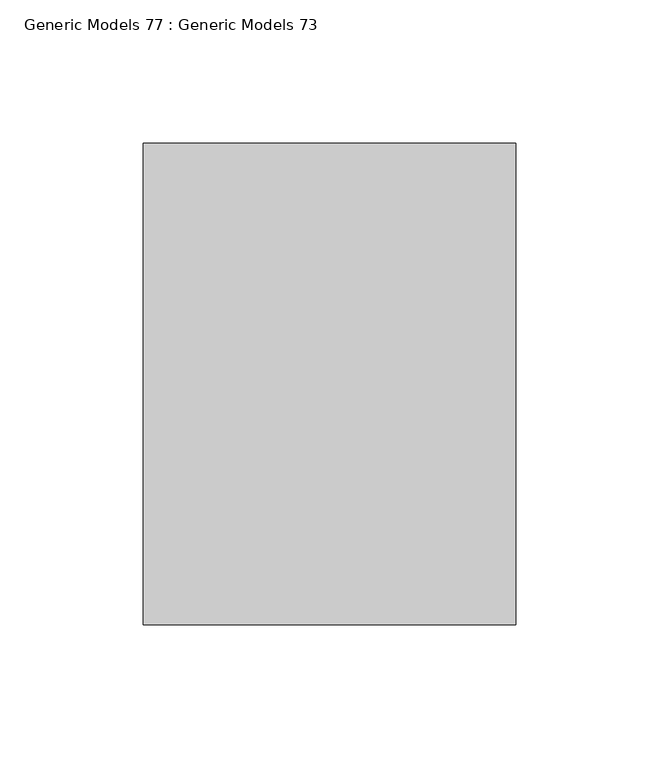
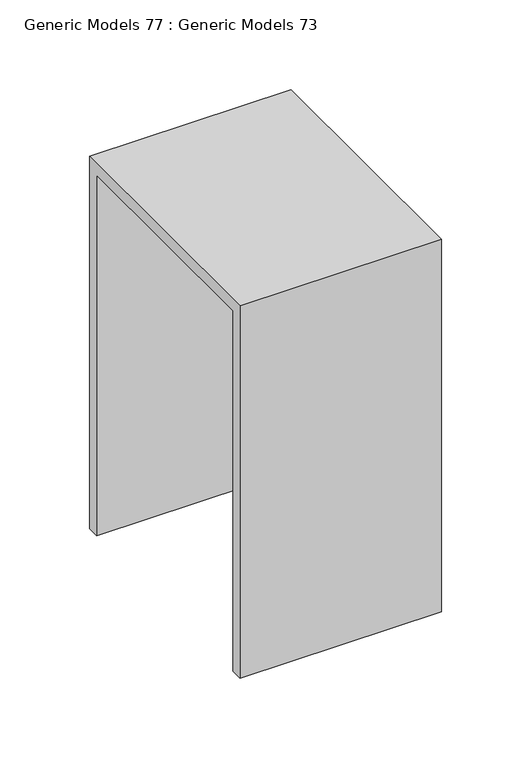
"""IFC4 building model written with IfcOpenShell, lengths in millimetres: proxy geometry, Generic Models 77 : Generic Models 73."""

import ifcopenshell
import ifcopenshell.guid

model = None  # the IFC model being written
_history = None  # IfcOwnerHistory: only IFC2X3 demands one
_inside = {}  # id of a spatial element -> (the spatial element, [elements in it])
_under = {}  # id of a project, library or spatial element -> (it, [spatial elements below it])
_declared = {}  # id of a project -> (the project, [libraries it declares])
_typed = {}  # id of a type object -> (the type object, [elements of that type])
_made_of = {}  # id of a material, layer set ... -> (it, [elements and type objects made of it])


def new_model(schema):
    """Start an empty IFC model of exactly this schema.

    Asked for "IFC4X3", IfcOpenShell would pick the latest addendum, in which some entities
    have other attributes; the version numbers below select the first issue.
    IFC2X3 requires an IfcOwnerHistory on every rooted entity: one is made here for all.
    """
    global model, _history
    if schema == "IFC4X3":
        model = ifcopenshell.file(schema_version=(4, 3, 0, 0))
    else:
        model = ifcopenshell.file(schema=schema)
    _inside.clear()
    _under.clear()
    _declared.clear()
    _typed.clear()
    _made_of.clear()
    _history = None
    if model.schema == "IFC2X3":
        org = make("IfcOrganization", Name="unknown")
        user = make(
            "IfcPersonAndOrganization",
            ThePerson=make("IfcPerson", FamilyName="unknown"),
            TheOrganization=org,
        )
        app = make(
            "IfcApplication",
            ApplicationDeveloper=org,
            Version="unknown",
            ApplicationFullName="unknown",
            ApplicationIdentifier="unknown",
        )
        _history = make(
            "IfcOwnerHistory",
            OwningUser=user,
            OwningApplication=app,
            ChangeAction="ADDED",
            CreationDate=0,
        )
    return model


def make(cls, **values):
    """One entity of the class cls with the attributes given. An attribute that is None is left unset."""
    return model.create_entity(
        cls, **{name: value for name, value in values.items() if value is not None}
    )


def rooted(cls, **values):
    """An entity with a GlobalId (a new one), such as an element, a storey or a relation."""
    return make(cls, GlobalId=ifcopenshell.guid.new(), OwnerHistory=_history, **values)


def si_unit(unit_type, name, prefix=None):
    """IfcSIUnit, for example si_unit("LENGTHUNIT", "METRE", prefix="MILLI")."""
    return make("IfcSIUnit", UnitType=unit_type, Prefix=prefix, Name=name)


def assignment(units):
    """IfcUnitAssignment: the units of a project."""
    return None if units is None else make("IfcUnitAssignment", Units=units)


def point(xyz):
    """IfcCartesianPoint."""
    return None if xyz is None else make("IfcCartesianPoint", Coordinates=xyz)


def direction(xyz):
    """IfcDirection."""
    return None if xyz is None else make("IfcDirection", DirectionRatios=xyz)


def frame(location, z_axis=None, x_axis=None):
    """IfcAxis2Placement3D, a coordinate frame: its origin and axes. An axis left out is left unset."""
    return make(
        "IfcAxis2Placement3D",
        Location=point(location),
        Axis=direction(z_axis),
        RefDirection=direction(x_axis),
    )


def origin():
    """The frame at (0, 0, 0) with its axes left unset."""
    return frame((0.0, 0.0, 0.0))


def place(relative_to, where):
    """IfcLocalPlacement: puts the frame where relative to a parent placement (None: the world)."""
    return make(
        "IfcLocalPlacement", PlacementRelTo=relative_to, RelativePlacement=where
    )


def context(
    kind, dimensions, precision=None, world=None, true_north=None, identifier=None
):
    """IfcGeometricRepresentationContext, for example the 3D "Model" context."""
    return make(
        "IfcGeometricRepresentationContext",
        ContextIdentifier=identifier,
        ContextType=kind,
        CoordinateSpaceDimension=dimensions,
        Precision=precision,
        WorldCoordinateSystem=world,
        TrueNorth=true_north,
    )


def project(units=None, contexts=None):
    """IfcProject with its units and contexts."""
    return rooted(
        "IfcProject",
        Name="project",
        RepresentationContexts=contexts,
        UnitsInContext=assignment(units),
    )


def spatial(cls, under=None, at=None, **own):
    """A site, building, storey or space (cls), placed at a placement, below another one or the project."""
    s = rooted(cls, ObjectPlacement=at, **own)
    if under is not None:
        _under.setdefault(under.id(), (under, []))[1].append(s)
    return s


def polyline(points):
    """IfcPolyline through the points."""
    return make("IfcPolyline", Points=[point(p) for p in points])


def outline(outer, holes=None, kind="AREA"):
    """IfcArbitraryClosedProfileDef: a profile drawn as a closed curve; with holes, ...WithVoids."""
    if holes is None:
        return make("IfcArbitraryClosedProfileDef", ProfileType=kind, OuterCurve=outer)
    return make(
        "IfcArbitraryProfileDefWithVoids",
        ProfileType=kind,
        OuterCurve=outer,
        InnerCurves=holes,
    )


def extrude(swept, where, along, depth):
    """IfcExtrudedAreaSolid: the profile swept, set in the frame where, extruded along a direction by depth."""
    return make(
        "IfcExtrudedAreaSolid",
        SweptArea=swept,
        Position=where,
        ExtrudedDirection=direction(along),
        Depth=depth,
    )


def shape(context_of_items, identifier, shape_type, items):
    """IfcShapeRepresentation: the items that make up one representation, for example the "Body"."""
    return make(
        "IfcShapeRepresentation",
        ContextOfItems=context_of_items,
        RepresentationIdentifier=identifier,
        RepresentationType=shape_type,
        Items=items,
    )


def source(mapping_origin, context_of_items, identifier, shape_type, items):
    """IfcRepresentationMap: a shape defined once, which mapped items show again and again."""
    return make(
        "IfcRepresentationMap",
        MappingOrigin=mapping_origin,
        MappedRepresentation=shape(context_of_items, identifier, shape_type, items),
    )


def transform(
    local_origin,
    x_axis=None,
    y_axis=None,
    z_axis=None,
    scale=None,
    scale2=None,
    scale3=None,
    uniform=True,
):
    """IfcCartesianTransformationOperator3D, or its non-uniform kind. x_axis, y_axis, z_axis: its Axis1, 2, 3."""
    if uniform:
        return make(
            "IfcCartesianTransformationOperator3D",
            Axis1=direction(x_axis),
            Axis2=direction(y_axis),
            LocalOrigin=point(local_origin),
            Scale=scale,
            Axis3=direction(z_axis),
        )
    return make(
        "IfcCartesianTransformationOperator3DnonUniform",
        Axis1=direction(x_axis),
        Axis2=direction(y_axis),
        LocalOrigin=point(local_origin),
        Scale=scale,
        Axis3=direction(z_axis),
        Scale2=scale2,
        Scale3=scale3,
    )


def mapped(mapping_source, mapping_target):
    """IfcMappedItem: shows the shape of a source again, moved by a transform."""
    return make(
        "IfcMappedItem", MappingSource=mapping_source, MappingTarget=mapping_target
    )


def made_of(thing, what):
    """Note that an element or type object is made of a material, layer set ...; save() writes the relation."""
    if what is not None:
        _made_of.setdefault(what.id(), (what, []))[1].append(thing)
    return thing


def element(
    cls,
    number,
    at=None,
    inside=None,
    cuts=None,
    type_object=None,
    material=None,
    context=None,
    identifier="Body",
    shape_type=None,
    held_by="IfcProductDefinitionShape",
    body=None,
    shapes=None,
    **own,
):
    """One element of the class cls, such as IfcWall. Its Tag is "e" and its number.

    at: its placement. inside: the storey or other place that contains it. cuts: it is an
    opening in that element (IfcRelVoidsElement). A single representation is given by context,
    identifier, shape_type and body (its items); several are given by shapes. held_by: the class
    of the entity that holds the representations. save() writes the other relations.
    """
    e = rooted(cls, Tag="e%d" % number, ObjectPlacement=at, **own)
    if body is not None:
        shapes = [shape(context, identifier, shape_type, body)]
    if shapes is not None:
        e.Representation = make(held_by, Representations=shapes)
    if inside is not None:
        _inside.setdefault(inside.id(), (inside, []))[1].append(e)
    if cuts is not None:
        rooted(
            "IfcRelVoidsElement", RelatingBuildingElement=cuts, RelatedOpeningElement=e
        )
    if type_object is not None:
        _typed.setdefault(type_object.id(), (type_object, []))[1].append(e)
    return made_of(e, material)


def aggregate(whole, parts):
    """IfcRelAggregates: a whole, such as a stair, and the parts it consists of."""
    return rooted("IfcRelAggregates", RelatingObject=whole, RelatedObjects=parts)


def save(model, path):
    """Write the relations noted so far, then the file.

    IfcRelAggregates (storeys below a building ...), IfcRelContainedInSpatialStructure (elements
    in a storey), IfcRelDefinesByType, IfcRelAssociatesMaterial and IfcRelDeclares: one each for
    every whole, place, type object, material and project.
    """
    for whole, parts in _under.values():
        aggregate(whole, parts)
    for where, things in _inside.values():
        rooted(
            "IfcRelContainedInSpatialStructure",
            RelatedElements=things,
            RelatingStructure=where,
        )
    for kind, things in _typed.values():
        rooted("IfcRelDefinesByType", RelatedObjects=things, RelatingType=kind)
    for what, things in _made_of.values():
        rooted("IfcRelAssociatesMaterial", RelatedObjects=things, RelatingMaterial=what)
    for by, libraries in _declared.values():
        rooted("IfcRelDeclares", RelatingContext=by, RelatedDefinitions=libraries)
    model.write(path)


def generic_models_77_generic_models_73_76b3ebb9(model_context):
    return source(origin(), model_context, "Body", "SweptSolid", [
        extrude(outline(polyline([(30850.5406612, 271462.5), (30698.1406612, 271462.5), (30698.1406612, 271216.4375), (30690.2031612, 271216.4375), (30690.2031612, 271470.4375), (30858.4781612, 271470.4375), (30858.4781612, 271216.4375), (30850.5406612, 271216.4375), (30850.5406612, 271462.5)])), frame((31910.3221032, 0.0, 0.0), z_axis=(1.0, 0.0, 0.0), x_axis=(0.0, 1.0, 0.0)), (0.0, 0.0, 1.0), 130.175),
    ])


if __name__ == "__main__":
    model = new_model("IFC4")
    model_context = context("Model", 3, world=origin())
    ifc_project = project(units=[si_unit("LENGTHUNIT", "METRE", prefix="MILLI")], contexts=[model_context])
    site = spatial("IfcSite", under=ifc_project)
    building = spatial("IfcBuilding", under=site)
    placement = place(None, origin())
    generic_models_77_generic_models_73_shape = generic_models_77_generic_models_73_76b3ebb9(model_context)
    element("IfcBuildingElementProxy", 1, Name="Generic Models 77 : Generic Models 73", ObjectType="Generic Models 77 : Generic Models 73", at=placement, inside=building, context=model_context, shape_type="MappedRepresentation", body=[
        mapped(generic_models_77_generic_models_73_shape, transform((0.0, 0.0, 0.0), x_axis=(1.0, 0.0, 0.0), y_axis=(0.0, 1.0, 0.0), z_axis=(0.0, 0.0, 1.0))),
    ])
    save(model, "model.ifc")

# Revit data of these elements
# Element 1 (IfcBuildingElementProxy, "Generic Models 77 : Generic Models 73")
#   Materials on its faces: "5/16 x5\" BENT PLATE CAP \nW/ 2 1\"DIA. THRU BOLTS"
# Materials
#   "5/16 x5\" BENT PLATE CAP \nW/ 2 1\"DIA. THRU BOLTS": class "Metal", colour RGB 199 199 199, transparency 0, Description = "Carbon steel", Cost = 0
